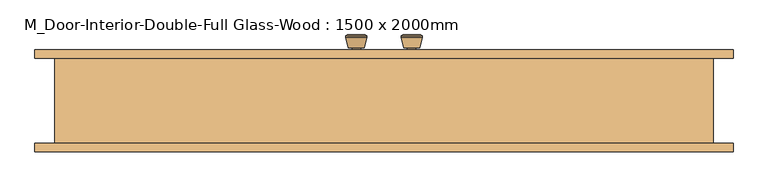
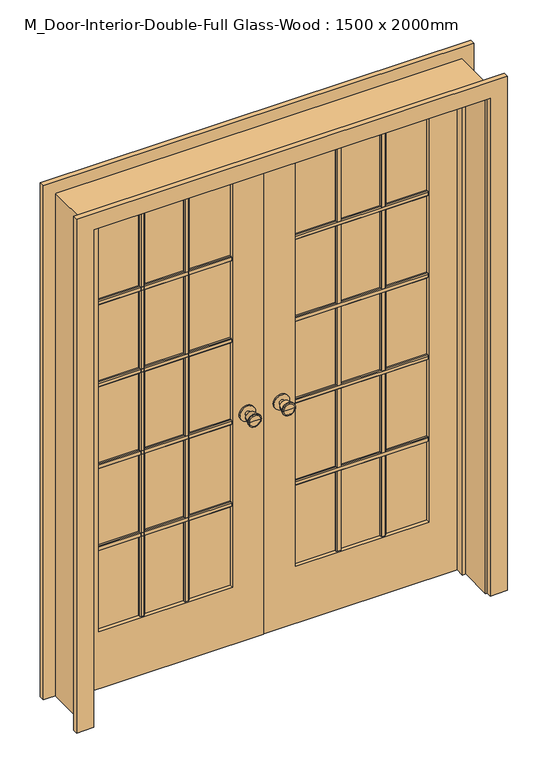
"""IFC4 building model written with IfcOpenShell, lengths in millimetres: door geometry, M_Door-Interior-Double-Full Glass-Wood : 1500 x 2000mm."""

import ifcopenshell
import ifcopenshell.guid

model = None  # the IFC model being written
_history = None  # IfcOwnerHistory: only IFC2X3 demands one
_inside = {}  # id of a spatial element -> (the spatial element, [elements in it])
_under = {}  # id of a project, library or spatial element -> (it, [spatial elements below it])
_declared = {}  # id of a project -> (the project, [libraries it declares])
_typed = {}  # id of a type object -> (the type object, [elements of that type])
_made_of = {}  # id of a material, layer set ... -> (it, [elements and type objects made of it])


def new_model(schema):
    """Start an empty IFC model of exactly this schema.

    Asked for "IFC4X3", IfcOpenShell would pick the latest addendum, in which some entities
    have other attributes; the version numbers below select the first issue.
    IFC2X3 requires an IfcOwnerHistory on every rooted entity: one is made here for all.
    """
    global model, _history
    if schema == "IFC4X3":
        model = ifcopenshell.file(schema_version=(4, 3, 0, 0))
    else:
        model = ifcopenshell.file(schema=schema)
    _inside.clear()
    _under.clear()
    _declared.clear()
    _typed.clear()
    _made_of.clear()
    _history = None
    if model.schema == "IFC2X3":
        org = make("IfcOrganization", Name="unknown")
        user = make(
            "IfcPersonAndOrganization",
            ThePerson=make("IfcPerson", FamilyName="unknown"),
            TheOrganization=org,
        )
        app = make(
            "IfcApplication",
            ApplicationDeveloper=org,
            Version="unknown",
            ApplicationFullName="unknown",
            ApplicationIdentifier="unknown",
        )
        _history = make(
            "IfcOwnerHistory",
            OwningUser=user,
            OwningApplication=app,
            ChangeAction="ADDED",
            CreationDate=0,
        )
    return model


def make(cls, **values):
    """One entity of the class cls with the attributes given. An attribute that is None is left unset."""
    return model.create_entity(
        cls, **{name: value for name, value in values.items() if value is not None}
    )


def rooted(cls, **values):
    """An entity with a GlobalId (a new one), such as an element, a storey or a relation."""
    return make(cls, GlobalId=ifcopenshell.guid.new(), OwnerHistory=_history, **values)


def si_unit(unit_type, name, prefix=None):
    """IfcSIUnit, for example si_unit("LENGTHUNIT", "METRE", prefix="MILLI")."""
    return make("IfcSIUnit", UnitType=unit_type, Prefix=prefix, Name=name)


def assignment(units):
    """IfcUnitAssignment: the units of a project."""
    return None if units is None else make("IfcUnitAssignment", Units=units)


def point(xyz):
    """IfcCartesianPoint."""
    return None if xyz is None else make("IfcCartesianPoint", Coordinates=xyz)


def direction(xyz):
    """IfcDirection."""
    return None if xyz is None else make("IfcDirection", DirectionRatios=xyz)


def frame(location, z_axis=None, x_axis=None):
    """IfcAxis2Placement3D, a coordinate frame: its origin and axes. An axis left out is left unset."""
    return make(
        "IfcAxis2Placement3D",
        Location=point(location),
        Axis=direction(z_axis),
        RefDirection=direction(x_axis),
    )


def frame_2d(location, x_axis=None):
    """IfcAxis2Placement2D, a coordinate frame in the plane: its origin and x axis."""
    return make(
        "IfcAxis2Placement2D", Location=point(location), RefDirection=direction(x_axis)
    )


def origin():
    """The frame at (0, 0, 0) with its axes left unset."""
    return frame((0.0, 0.0, 0.0))


def place(relative_to, where):
    """IfcLocalPlacement: puts the frame where relative to a parent placement (None: the world)."""
    return make(
        "IfcLocalPlacement", PlacementRelTo=relative_to, RelativePlacement=where
    )


def context(
    kind, dimensions, precision=None, world=None, true_north=None, identifier=None
):
    """IfcGeometricRepresentationContext, for example the 3D "Model" context."""
    return make(
        "IfcGeometricRepresentationContext",
        ContextIdentifier=identifier,
        ContextType=kind,
        CoordinateSpaceDimension=dimensions,
        Precision=precision,
        WorldCoordinateSystem=world,
        TrueNorth=true_north,
    )


def project(units=None, contexts=None):
    """IfcProject with its units and contexts."""
    return rooted(
        "IfcProject",
        Name="project",
        RepresentationContexts=contexts,
        UnitsInContext=assignment(units),
    )


def spatial(cls, under=None, at=None, **own):
    """A site, building, storey or space (cls), placed at a placement, below another one or the project."""
    s = rooted(cls, ObjectPlacement=at, **own)
    if under is not None:
        _under.setdefault(under.id(), (under, []))[1].append(s)
    return s


def polyline(points):
    """IfcPolyline through the points."""
    return make("IfcPolyline", Points=[point(p) for p in points])


def circle_curve(where, radius):
    """IfcCircle in the frame where."""
    return make("IfcCircle", Position=where, Radius=radius)


def trimmed(basis, trim1, trim2, sense, master):
    """IfcTrimmedCurve: the piece of a basis curve between two trims."""
    return make(
        "IfcTrimmedCurve",
        BasisCurve=basis,
        Trim1=trim1,
        Trim2=trim2,
        SenseAgreement=sense,
        MasterRepresentation=master,
    )


def segment(curve, same_sense, transition):
    """IfcCompositeCurveSegment."""
    return make(
        "IfcCompositeCurveSegment",
        Transition=transition,
        SameSense=same_sense,
        ParentCurve=curve,
    )


def composite_curve(segments, self_intersect=None):
    """IfcCompositeCurve: segments joined end to end."""
    return make("IfcCompositeCurve", Segments=segments, SelfIntersect=self_intersect)


def outline(outer, holes=None, kind="AREA"):
    """IfcArbitraryClosedProfileDef: a profile drawn as a closed curve; with holes, ...WithVoids."""
    if holes is None:
        return make("IfcArbitraryClosedProfileDef", ProfileType=kind, OuterCurve=outer)
    return make(
        "IfcArbitraryProfileDefWithVoids",
        ProfileType=kind,
        OuterCurve=outer,
        InnerCurves=holes,
    )


def extrude(swept, where, along, depth):
    """IfcExtrudedAreaSolid: the profile swept, set in the frame where, extruded along a direction by depth."""
    return make(
        "IfcExtrudedAreaSolid",
        SweptArea=swept,
        Position=where,
        ExtrudedDirection=direction(along),
        Depth=depth,
    )


def faces_of(points, faces, orient=None, outer=None):
    """IfcFace entities. A face is a list of loops; a loop is a list of indices into points, from 0.

    orient and outer hold one flag for each loop. By default every Orientation is true, the
    first loop of a face is its IfcFaceOuterBound and the others are IfcFaceBound.
    """
    made = []
    for i, loops in enumerate(faces):
        bounds = []
        for j, loop in enumerate(loops):
            is_outer = j == 0 if outer is None else outer[i][j]
            bounds.append(
                make(
                    "IfcFaceOuterBound" if is_outer else "IfcFaceBound",
                    Bound=make("IfcPolyLoop", Polygon=[points[k] for k in loop]),
                    Orientation=True if orient is None else orient[i][j],
                )
            )
        made.append(make("IfcFace", Bounds=bounds))
    return made


def faceted_brep(points, faces, orient=None, outer=None, voids=None):
    """IfcFacetedBrep: a solid bounded by flat faces; with voids (closed shells), ...WithVoids."""
    shared = [point(p) for p in points]
    hull = make("IfcClosedShell", CfsFaces=faces_of(shared, faces, orient, outer))
    if voids is None:
        return make("IfcFacetedBrep", Outer=hull)
    return make(
        "IfcFacetedBrepWithVoids",
        Outer=hull,
        Voids=[
            make(cls, CfsFaces=faces_of(shared, fs, o, b)) for cls, fs, o, b in voids
        ],
    )


def shape(context_of_items, identifier, shape_type, items):
    """IfcShapeRepresentation: the items that make up one representation, for example the "Body"."""
    return make(
        "IfcShapeRepresentation",
        ContextOfItems=context_of_items,
        RepresentationIdentifier=identifier,
        RepresentationType=shape_type,
        Items=items,
    )


def source(mapping_origin, context_of_items, identifier, shape_type, items):
    """IfcRepresentationMap: a shape defined once, which mapped items show again and again."""
    return make(
        "IfcRepresentationMap",
        MappingOrigin=mapping_origin,
        MappedRepresentation=shape(context_of_items, identifier, shape_type, items),
    )


def transform(
    local_origin,
    x_axis=None,
    y_axis=None,
    z_axis=None,
    scale=None,
    scale2=None,
    scale3=None,
    uniform=True,
):
    """IfcCartesianTransformationOperator3D, or its non-uniform kind. x_axis, y_axis, z_axis: its Axis1, 2, 3."""
    if uniform:
        return make(
            "IfcCartesianTransformationOperator3D",
            Axis1=direction(x_axis),
            Axis2=direction(y_axis),
            LocalOrigin=point(local_origin),
            Scale=scale,
            Axis3=direction(z_axis),
        )
    return make(
        "IfcCartesianTransformationOperator3DnonUniform",
        Axis1=direction(x_axis),
        Axis2=direction(y_axis),
        LocalOrigin=point(local_origin),
        Scale=scale,
        Axis3=direction(z_axis),
        Scale2=scale2,
        Scale3=scale3,
    )


def mapped(mapping_source, mapping_target):
    """IfcMappedItem: shows the shape of a source again, moved by a transform."""
    return make(
        "IfcMappedItem", MappingSource=mapping_source, MappingTarget=mapping_target
    )


def made_of(thing, what):
    """Note that an element or type object is made of a material, layer set ...; save() writes the relation."""
    if what is not None:
        _made_of.setdefault(what.id(), (what, []))[1].append(thing)
    return thing


def element(
    cls,
    number,
    at=None,
    inside=None,
    cuts=None,
    type_object=None,
    material=None,
    context=None,
    identifier="Body",
    shape_type=None,
    held_by="IfcProductDefinitionShape",
    body=None,
    shapes=None,
    **own,
):
    """One element of the class cls, such as IfcWall. Its Tag is "e" and its number.

    at: its placement. inside: the storey or other place that contains it. cuts: it is an
    opening in that element (IfcRelVoidsElement). A single representation is given by context,
    identifier, shape_type and body (its items); several are given by shapes. held_by: the class
    of the entity that holds the representations. save() writes the other relations.
    """
    e = rooted(cls, Tag="e%d" % number, ObjectPlacement=at, **own)
    if body is not None:
        shapes = [shape(context, identifier, shape_type, body)]
    if shapes is not None:
        e.Representation = make(held_by, Representations=shapes)
    if inside is not None:
        _inside.setdefault(inside.id(), (inside, []))[1].append(e)
    if cuts is not None:
        rooted(
            "IfcRelVoidsElement", RelatingBuildingElement=cuts, RelatedOpeningElement=e
        )
    if type_object is not None:
        _typed.setdefault(type_object.id(), (type_object, []))[1].append(e)
    return made_of(e, material)


def aggregate(whole, parts):
    """IfcRelAggregates: a whole, such as a stair, and the parts it consists of."""
    return rooted("IfcRelAggregates", RelatingObject=whole, RelatedObjects=parts)


def save(model, path):
    """Write the relations noted so far, then the file.

    IfcRelAggregates (storeys below a building ...), IfcRelContainedInSpatialStructure (elements
    in a storey), IfcRelDefinesByType, IfcRelAssociatesMaterial and IfcRelDeclares: one each for
    every whole, place, type object, material and project.
    """
    for whole, parts in _under.values():
        aggregate(whole, parts)
    for where, things in _inside.values():
        rooted(
            "IfcRelContainedInSpatialStructure",
            RelatedElements=things,
            RelatingStructure=where,
        )
    for kind, things in _typed.values():
        rooted("IfcRelDefinesByType", RelatedObjects=things, RelatingType=kind)
    for what, things in _made_of.values():
        rooted("IfcRelAssociatesMaterial", RelatedObjects=things, RelatingMaterial=what)
    for by, libraries in _declared.values():
        rooted("IfcRelDeclares", RelatingContext=by, RelatedDefinitions=libraries)
    model.write(path)


def plane_surface(at):
    """IfcPlane: the flat surface through the origin of the frame at, square to its z axis."""
    return make("IfcPlane", Position=at)


def cylinder_surface(at, radius):
    """IfcCylindricalSurface: all points at the distance radius from the z axis of the frame at."""
    return make("IfcCylindricalSurface", Position=at, Radius=radius)


def revolved_surface(curve, axis_point, axis_direction):
    """IfcSurfaceOfRevolution: the curve turned about the line through axis_point along axis_direction."""
    return make(
        "IfcSurfaceOfRevolution",
        SweptCurve=make("IfcArbitraryOpenProfileDef", ProfileType="CURVE", Curve=curve),
        AxisPosition=make("IfcAxis1Placement", Location=point(axis_point), Axis=direction(axis_direction)),
    )


def advanced_brep(points, edges, surfaces, faces):
    """IfcAdvancedBrep: a solid bounded by faces that lie on surfaces and meet in shared edges.

    An edge is (start, end): straight between two places in points (the first is 0);
    or (start, end, curve); or (start, end, curve, False) where it runs against its curve.
    A face is (place in surfaces, loops), or (place, loops, False) where it looks against
    its surface's normal. A loop lists edges by number (the first is 1), with a minus sign
    where the edge is run from its end to its start. The first loop is the outer one.
    """
    corners = [point(p) for p in points]
    vertices = [make("IfcVertexPoint", VertexGeometry=c) for c in corners]
    made = []
    for start, end, *more in edges:
        made.append(
            make(
                "IfcEdgeCurve",
                EdgeStart=vertices[start],
                EdgeEnd=vertices[end],
                EdgeGeometry=more[0] if more else make("IfcPolyline", Points=[corners[start], corners[end]]),
                SameSense=more[1] if len(more) > 1 else True,
            )
        )
    hull = []
    for where, loops, *sense in faces:
        bounds = []
        for j, loop in enumerate(loops):
            ring = [make("IfcOrientedEdge", EdgeElement=made[abs(k) - 1], Orientation=k > 0) for k in loop]
            bounds.append(
                make(
                    "IfcFaceOuterBound" if j == 0 else "IfcFaceBound",
                    Bound=make("IfcEdgeLoop", EdgeList=ring),
                    Orientation=True,
                )
            )
        hull.append(make("IfcAdvancedFace", Bounds=bounds, FaceSurface=surfaces[where], SameSense=sense[0] if sense else True))
    return make("IfcAdvancedBrep", Outer=make("IfcClosedShell", CfsFaces=hull))


def m_door_interior_double_full_glass_wood_1500_x_2000mm_af437330(model_context):
    return source(origin(), model_context, "Body", "SolidModel", [
        advanced_brep(
        [(-65.0, 102.825, 914.4), (-75.0, 102.825, 914.4), (-55.0, 102.825, 914.4), (-85.4758676, 151.825, 914.4), (-65.0, 151.825, 914.4), (-44.5241324, 151.825, 914.4), (-90.0, 149.9971319, 914.4), (-40.0, 149.9971319, 914.4), (-90.0, 146.5334537, 914.4), (-40.0, 146.5334537, 914.4), (-83.636236, 121.825, 914.4), (-46.363764, 121.825, 914.4), (-75.0, 121.825, 914.4), (-55.0, 121.825, 914.4)],
        [
            (0, 1),
            (1, 2, circle_curve(frame((-65.0, 102.825, 914.4), z_axis=(0.0, -1.0, 0.0), x_axis=(1.0, 0.0, 0.0)), 10.0)),
            (2, 0),
            (2, 1, circle_curve(frame((-65.0, 102.825, 914.4), z_axis=(0.0, -1.0, 0.0), x_axis=(1.0, 0.0, 0.0)), 10.0)),
            (3, 4),
            (4, 5),
            (5, 3, circle_curve(frame((-65.0, 151.825, 914.4), z_axis=(0.0, 1.0, 0.0), x_axis=(1.0, 0.0, 0.0)), 20.4758676)),
            (3, 5, circle_curve(frame((-65.0, 151.825, 914.4), z_axis=(0.0, 1.0, 0.0), x_axis=(1.0, 0.0, 0.0)), 20.4758676)),
            (6, 3),
            (5, 7),
            (7, 6, circle_curve(frame((-65.0, 149.9971319, 914.4), z_axis=(0.0, 1.0, 0.0), x_axis=(1.0, 0.0, 0.0)), 25.0)),
            (6, 7, circle_curve(frame((-65.0, 149.9971319, 914.4), z_axis=(0.0, 1.0, 0.0), x_axis=(1.0, 0.0, 0.0)), 25.0)),
            (8, 6),
            (7, 9),
            (9, 8, circle_curve(frame((-65.0, 146.5334537, 914.4), z_axis=(0.0, 1.0, 0.0), x_axis=(1.0, 0.0, 0.0)), 25.0)),
            (8, 9, circle_curve(frame((-65.0, 146.5334537, 914.4), z_axis=(0.0, 1.0, 0.0), x_axis=(1.0, 0.0, 0.0)), 25.0)),
            (10, 8),
            (9, 11),
            (11, 10, circle_curve(frame((-65.0, 121.825, 914.4), z_axis=(0.0, 1.0, 0.0), x_axis=(1.0, 0.0, 0.0)), 18.636236)),
            (10, 11, circle_curve(frame((-65.0, 121.825, 914.4), z_axis=(0.0, 1.0, 0.0), x_axis=(1.0, 0.0, 0.0)), 18.636236)),
            (12, 10),
            (11, 13),
            (13, 12, circle_curve(frame((-65.0, 121.825, 914.4), z_axis=(0.0, 1.0, 0.0), x_axis=(1.0, 0.0, 0.0)), 10.0)),
            (12, 13, circle_curve(frame((-65.0, 121.825, 914.4), z_axis=(0.0, 1.0, 0.0), x_axis=(1.0, 0.0, 0.0)), 10.0)),
            (1, 12),
            (13, 2),
        ],
        [
            plane_surface(frame((-65.0, 102.825, 914.4), z_axis=(0.0, -1.0, 0.0), x_axis=(1.0, 0.0, 0.0))),
            plane_surface(frame((-65.0, 151.825, 914.4), z_axis=(0.0, 1.0, 0.0), x_axis=(1.0, 0.0, 0.0))),
            revolved_surface(polyline([(-44.5241324, 151.825, 914.4), (-40.0, 149.9971319, 914.4)]), (-65.0, 102.825, 914.4), (0.0, -1.0, 0.0)),
            cylinder_surface(frame((-65.0, 102.825, 914.4), z_axis=(0.0, -1.0, 0.0), x_axis=(1.0, 0.0, 0.0)), 25.0),
            revolved_surface(polyline([(-40.0, 146.5334537, 914.4), (-46.363764, 121.825, 914.4)]), (-65.0, 102.825, 914.4), (0.0, -1.0, 0.0)),
            plane_surface(frame((-65.0, 121.825, 914.4), z_axis=(0.0, -1.0, 0.0), x_axis=(1.0, 0.0, 0.0))),
            cylinder_surface(frame((-65.0, 102.825, 914.4), z_axis=(0.0, -1.0, 0.0), x_axis=(1.0, 0.0, 0.0)), 10.0),
        ],
        [
            (0, [[1, 2, 3]]),
            (0, [[-3, 4, -1]]),
            (1, [[5, 6, 7]]),
            (1, [[-6, -5, 8]]),
            (2, [[9, -7, 10, 11]]),
            (2, [[-10, -8, -9, 12]]),
            (3, [[13, -11, 14, 15]]),
            (3, [[-14, -12, -13, 16]]),
            (4, [[17, -15, 18, 19]]),
            (4, [[-18, -16, -17, 20]]),
            (5, [[21, -19, 22, 23]]),
            (5, [[-22, -20, -21, 24]]),
            (6, [[25, -23, 26, -2]]),
            (6, [[-26, -24, -25, -4]]),
        ],
    ),
        extrude(outline(composite_curve([segment(trimmed(circle_curve(frame_2d((914.4, -65.0)), 30.0), [point((914.4, -35.0))], [point((914.4, -95.0))], False, "CARTESIAN"), True, "CONTINUOUS"), segment(trimmed(circle_curve(frame_2d((914.4, -65.0)), 30.0), [point((914.4, -95.0))], [point((914.4, -35.0))], False, "CARTESIAN"), True, "CONTINUOUS")], self_intersect=False)), frame((0.0, 96.825, 0.0), z_axis=(0.0, 1.0, 0.0), x_axis=(0.0, 0.0, 1.0)), (0.0, 0.0, 1.0), 6.0),
        advanced_brep(
        [(-65.0, 55.825, 914.4), (-55.0, 55.825, 914.4), (-75.0, 55.825, 914.4), (-85.4758676, 6.825, 914.4), (-44.5241324, 6.825, 914.4), (-65.0, 6.825, 914.4), (-90.0, 8.6528681, 914.4), (-40.0, 8.6528681, 914.4), (-90.0, 12.1165463, 914.4), (-40.0, 12.1165463, 914.4), (-83.636236, 36.825, 914.4), (-46.363764, 36.825, 914.4), (-75.0, 36.825, 914.4), (-55.0, 36.825, 914.4)],
        [
            (0, 1),
            (1, 2, circle_curve(frame((-65.0, 55.825, 914.4), z_axis=(0.0, 1.0, 0.0), x_axis=(1.0, 0.0, 0.0)), 10.0)),
            (2, 0),
            (2, 1, circle_curve(frame((-65.0, 55.825, 914.4), z_axis=(0.0, 1.0, 0.0), x_axis=(1.0, 0.0, 0.0)), 10.0)),
            (3, 4, circle_curve(frame((-65.0, 6.825, 914.4), z_axis=(0.0, -1.0, 0.0), x_axis=(1.0, 0.0, 0.0)), 20.4758676)),
            (4, 5),
            (5, 3),
            (4, 3, circle_curve(frame((-65.0, 6.825, 914.4), z_axis=(0.0, -1.0, 0.0), x_axis=(1.0, 0.0, 0.0)), 20.4758676)),
            (6, 7, circle_curve(frame((-65.0, 8.6528681, 914.4), z_axis=(0.0, -1.0, 0.0), x_axis=(1.0, 0.0, 0.0)), 25.0)),
            (7, 4),
            (3, 6),
            (7, 6, circle_curve(frame((-65.0, 8.6528681, 914.4), z_axis=(0.0, -1.0, 0.0), x_axis=(1.0, 0.0, 0.0)), 25.0)),
            (8, 9, circle_curve(frame((-65.0, 12.1165463, 914.4), z_axis=(0.0, -1.0, 0.0), x_axis=(1.0, 0.0, 0.0)), 25.0)),
            (9, 7),
            (6, 8),
            (9, 8, circle_curve(frame((-65.0, 12.1165463, 914.4), z_axis=(0.0, -1.0, 0.0), x_axis=(1.0, 0.0, 0.0)), 25.0)),
            (10, 11, circle_curve(frame((-65.0, 36.825, 914.4), z_axis=(0.0, -1.0, 0.0), x_axis=(1.0, 0.0, 0.0)), 18.636236)),
            (11, 9),
            (8, 10),
            (11, 10, circle_curve(frame((-65.0, 36.825, 914.4), z_axis=(0.0, -1.0, 0.0), x_axis=(1.0, 0.0, 0.0)), 18.636236)),
            (12, 13, circle_curve(frame((-65.0, 36.825, 914.4), z_axis=(0.0, -1.0, 0.0), x_axis=(1.0, 0.0, 0.0)), 10.0)),
            (13, 11),
            (10, 12),
            (13, 12, circle_curve(frame((-65.0, 36.825, 914.4), z_axis=(0.0, -1.0, 0.0), x_axis=(1.0, 0.0, 0.0)), 10.0)),
            (1, 13),
            (12, 2),
        ],
        [
            plane_surface(frame((-65.0, 55.825, 914.4), z_axis=(0.0, 1.0, 0.0), x_axis=(1.0, 0.0, 0.0))),
            plane_surface(frame((-65.0, 6.825, 914.4), z_axis=(0.0, -1.0, 0.0), x_axis=(1.0, 0.0, 0.0))),
            revolved_surface(polyline([(-44.5241324, 6.825, 914.4), (-40.0, 8.6528681, 914.4)]), (-65.0, 55.825, 914.4), (0.0, 1.0, 0.0)),
            cylinder_surface(frame((-65.0, 55.825, 914.4), z_axis=(0.0, 1.0, 0.0), x_axis=(1.0, 0.0, 0.0)), 25.0),
            revolved_surface(polyline([(-40.0, 12.1165463, 914.4), (-46.363764, 36.825, 914.4)]), (-65.0, 55.825, 914.4), (0.0, 1.0, 0.0)),
            plane_surface(frame((-65.0, 36.825, 914.4), z_axis=(0.0, 1.0, 0.0), x_axis=(1.0, 0.0, 0.0))),
            cylinder_surface(frame((-65.0, 55.825, 914.4), z_axis=(0.0, 1.0, 0.0), x_axis=(1.0, 0.0, 0.0)), 10.0),
        ],
        [
            (0, [[1, 2, 3]]),
            (0, [[-3, 4, -1]]),
            (1, [[5, 6, 7]]),
            (1, [[8, -7, -6]]),
            (2, [[9, 10, -5, 11]]),
            (2, [[12, -11, -8, -10]]),
            (3, [[13, 14, -9, 15]]),
            (3, [[16, -15, -12, -14]]),
            (4, [[17, 18, -13, 19]]),
            (4, [[20, -19, -16, -18]]),
            (5, [[21, 22, -17, 23]]),
            (5, [[24, -23, -20, -22]]),
            (6, [[-2, 25, -21, 26]]),
            (6, [[-4, -26, -24, -25]]),
        ],
    ),
        extrude(outline(composite_curve([segment(trimmed(circle_curve(frame_2d((914.4, -65.0)), 30.0), [point((914.4, -35.0))], [point((914.4, -95.0))], False, "CARTESIAN"), True, "CONTINUOUS"), segment(trimmed(circle_curve(frame_2d((914.4, -65.0)), 30.0), [point((914.4, -95.0))], [point((914.4, -35.0))], False, "CARTESIAN"), True, "CONTINUOUS")], self_intersect=False)), frame((0.0, 55.825, 0.0), z_axis=(0.0, 1.0, 0.0), x_axis=(0.0, 0.0, 1.0)), (0.0, 0.0, 1.0), 6.0),
        extrude(outline(polyline([(75.825, 1559.525), (75.825, 1540.475), (69.475, 1540.475), (66.3, 1543.65), (66.3, 1556.35), (69.475, 1559.525), (75.825, 1559.525)])), frame((120.0, 0.0, 0.0), z_axis=(1.0, 0.0, 0.0), x_axis=(0.0, 1.0, 0.0)), (0.0, 0.0, 1.0), 510.0),
        extrude(outline(polyline([(75.825, 1229.525), (75.825, 1210.475), (69.475, 1210.475), (66.3, 1213.65), (66.3, 1226.35), (69.475, 1229.525), (75.825, 1229.525)])), frame((120.0, 0.0, 0.0), z_axis=(1.0, 0.0, 0.0), x_axis=(0.0, 1.0, 0.0)), (0.0, 0.0, 1.0), 510.0),
        extrude(outline(polyline([(75.825, 899.525), (75.825, 880.475), (69.475, 880.475), (66.3, 883.65), (66.3, 896.35), (69.475, 899.525), (75.825, 899.525)])), frame((120.0, 0.0, 0.0), z_axis=(1.0, 0.0, 0.0), x_axis=(0.0, 1.0, 0.0)), (0.0, 0.0, 1.0), 510.0),
        extrude(outline(polyline([(75.825, 569.525), (75.825, 550.475), (69.475, 550.475), (66.3, 553.65), (66.3, 566.35), (69.475, 569.525), (75.825, 569.525)])), frame((120.0, 0.0, 0.0), z_axis=(1.0, 0.0, 0.0), x_axis=(0.0, 1.0, 0.0)), (0.0, 0.0, 1.0), 510.0),
        extrude(outline(polyline([(450.475, 75.825), (469.525, 75.825), (469.525, 69.475), (466.35, 66.3), (453.65, 66.3), (450.475, 69.475), (450.475, 75.825)])), frame((0.0, 0.0, 230.0), z_axis=(0.0, 0.0, 1.0), x_axis=(1.0, 0.0, 0.0)), (0.0, 0.0, 1.0), 1650.0),
        extrude(outline(polyline([(280.475, 75.825), (299.525, 75.825), (299.525, 69.475), (296.35, 66.3), (283.65, 66.3), (280.475, 69.475), (280.475, 75.825)])), frame((0.0, 0.0, 230.0), z_axis=(0.0, 0.0, 1.0), x_axis=(1.0, 0.0, 0.0)), (0.0, 0.0, 1.0), 1650.0),
        extrude(outline(polyline([(82.825, 1559.525), (89.175, 1559.525), (92.35, 1556.35), (92.35, 1543.65), (89.175, 1540.475), (82.825, 1540.475), (82.825, 1559.525)])), frame((-630.0, 0.0, 0.0), z_axis=(1.0, 0.0, 0.0), x_axis=(0.0, 1.0, 0.0)), (0.0, 0.0, 1.0), 510.0),
        extrude(outline(polyline([(82.825, 1229.525), (89.175, 1229.525), (92.35, 1226.35), (92.35, 1213.65), (89.175, 1210.475), (82.825, 1210.475), (82.825, 1229.525)])), frame((-630.0, 0.0, 0.0), z_axis=(1.0, 0.0, 0.0), x_axis=(0.0, 1.0, 0.0)), (0.0, 0.0, 1.0), 510.0),
        extrude(outline(polyline([(82.825, 899.525), (89.175, 899.525), (92.35, 896.35), (92.35, 883.65), (89.175, 880.475), (82.825, 880.475), (82.825, 899.525)])), frame((-630.0, 0.0, 0.0), z_axis=(1.0, 0.0, 0.0), x_axis=(0.0, 1.0, 0.0)), (0.0, 0.0, 1.0), 510.0),
        extrude(outline(polyline([(82.825, 569.525), (89.175, 569.525), (92.35, 566.35), (92.35, 553.65), (89.175, 550.475), (82.825, 550.475), (82.825, 569.525)])), frame((-630.0, 0.0, 0.0), z_axis=(1.0, 0.0, 0.0), x_axis=(0.0, 1.0, 0.0)), (0.0, 0.0, 1.0), 510.0),
        extrude(outline(polyline([(-299.525, 82.825), (-299.525, 89.175), (-296.35, 92.35), (-283.65, 92.35), (-280.475, 89.175), (-280.475, 82.825), (-299.525, 82.825)])), frame((0.0, 0.0, 230.0), z_axis=(0.0, 0.0, 1.0), x_axis=(1.0, 0.0, 0.0)), (0.0, 0.0, 1.0), 1650.0),
        extrude(outline(polyline([(-469.525, 82.825), (-469.525, 89.175), (-466.35, 92.35), (-453.65, 92.35), (-450.475, 89.175), (-450.475, 82.825), (-469.525, 82.825)])), frame((0.0, 0.0, 230.0), z_axis=(0.0, 0.0, 1.0), x_axis=(1.0, 0.0, 0.0)), (0.0, 0.0, 1.0), 1650.0),
        extrude(outline(polyline([(82.825, 1559.525), (89.175, 1559.525), (92.35, 1556.35), (92.35, 1543.65), (89.175, 1540.475), (82.825, 1540.475), (82.825, 1559.525)])), frame((120.0, 0.0, 0.0), z_axis=(1.0, 0.0, 0.0), x_axis=(0.0, 1.0, 0.0)), (0.0, 0.0, 1.0), 510.0),
        extrude(outline(polyline([(82.825, 1229.525), (89.175, 1229.525), (92.35, 1226.35), (92.35, 1213.65), (89.175, 1210.475), (82.825, 1210.475), (82.825, 1229.525)])), frame((120.0, 0.0, 0.0), z_axis=(1.0, 0.0, 0.0), x_axis=(0.0, 1.0, 0.0)), (0.0, 0.0, 1.0), 510.0),
        extrude(outline(polyline([(82.825, 899.525), (89.175, 899.525), (92.35, 896.35), (92.35, 883.65), (89.175, 880.475), (82.825, 880.475), (82.825, 899.525)])), frame((120.0, 0.0, 0.0), z_axis=(1.0, 0.0, 0.0), x_axis=(0.0, 1.0, 0.0)), (0.0, 0.0, 1.0), 510.0),
        extrude(outline(polyline([(82.825, 569.525), (89.175, 569.525), (92.35, 566.35), (92.35, 553.65), (89.175, 550.475), (82.825, 550.475), (82.825, 569.525)])), frame((120.0, 0.0, 0.0), z_axis=(1.0, 0.0, 0.0), x_axis=(0.0, 1.0, 0.0)), (0.0, 0.0, 1.0), 510.0),
        extrude(outline(polyline([(450.475, 82.825), (450.475, 89.175), (453.65, 92.35), (466.35, 92.35), (469.525, 89.175), (469.525, 82.825), (450.475, 82.825)])), frame((0.0, 0.0, 230.0), z_axis=(0.0, 0.0, 1.0), x_axis=(1.0, 0.0, 0.0)), (0.0, 0.0, 1.0), 1650.0),
        extrude(outline(polyline([(280.475, 82.825), (280.475, 89.175), (283.65, 92.35), (296.35, 92.35), (299.525, 89.175), (299.525, 82.825), (280.475, 82.825)])), frame((0.0, 0.0, 230.0), z_axis=(0.0, 0.0, 1.0), x_axis=(1.0, 0.0, 0.0)), (0.0, 0.0, 1.0), 1650.0),
        extrude(outline(polyline([(75.825, 1559.525), (75.825, 1540.475), (69.475, 1540.475), (66.3, 1543.65), (66.3, 1556.35), (69.475, 1559.525), (75.825, 1559.525)])), frame((-630.0, 0.0, 0.0), z_axis=(1.0, 0.0, 0.0), x_axis=(0.0, 1.0, 0.0)), (0.0, 0.0, 1.0), 510.0),
        extrude(outline(polyline([(75.825, 1229.525), (75.825, 1210.475), (69.475, 1210.475), (66.3, 1213.65), (66.3, 1226.35), (69.475, 1229.525), (75.825, 1229.525)])), frame((-630.0, 0.0, 0.0), z_axis=(1.0, 0.0, 0.0), x_axis=(0.0, 1.0, 0.0)), (0.0, 0.0, 1.0), 510.0),
        extrude(outline(polyline([(75.825, 899.525), (75.825, 880.475), (69.475, 880.475), (66.3, 883.65), (66.3, 896.35), (69.475, 899.525), (75.825, 899.525)])), frame((-630.0, 0.0, 0.0), z_axis=(1.0, 0.0, 0.0), x_axis=(0.0, 1.0, 0.0)), (0.0, 0.0, 1.0), 510.0),
        extrude(outline(polyline([(75.825, 569.525), (75.825, 550.475), (69.475, 550.475), (66.3, 553.65), (66.3, 566.35), (69.475, 569.525), (75.825, 569.525)])), frame((-630.0, 0.0, 0.0), z_axis=(1.0, 0.0, 0.0), x_axis=(0.0, 1.0, 0.0)), (0.0, 0.0, 1.0), 510.0),
        extrude(outline(polyline([(-299.525, 75.825), (-280.475, 75.825), (-280.475, 69.475), (-283.65, 66.3), (-296.35, 66.3), (-299.525, 69.475), (-299.525, 75.825)])), frame((0.0, 0.0, 230.0), z_axis=(0.0, 0.0, 1.0), x_axis=(1.0, 0.0, 0.0)), (0.0, 0.0, 1.0), 1650.0),
        extrude(outline(polyline([(-469.525, 75.825), (-450.475, 75.825), (-450.475, 69.475), (-453.65, 66.3), (-466.35, 66.3), (-469.525, 69.475), (-469.525, 75.825)])), frame((0.0, 0.0, 230.0), z_axis=(0.0, 0.0, 1.0), x_axis=(1.0, 0.0, 0.0)), (0.0, 0.0, 1.0), 1650.0),
        advanced_brep(
        [(65.0, 55.825, 914.4), (75.0, 55.825, 914.4), (55.0, 55.825, 914.4), (85.4758676, 6.825, 914.4), (65.0, 6.825, 914.4), (44.5241324, 6.825, 914.4), (90.0, 8.6528681, 914.4), (40.0, 8.6528681, 914.4), (90.0, 12.1165463, 914.4), (40.0, 12.1165463, 914.4), (83.636236, 36.825, 914.4), (46.363764, 36.825, 914.4), (75.0, 36.825, 914.4), (55.0, 36.825, 914.4)],
        [
            (0, 1),
            (1, 2, circle_curve(frame((65.0, 55.825, 914.4), z_axis=(0.0, 1.0, 0.0), x_axis=(-1.0, 0.0, 0.0)), 10.0)),
            (2, 0),
            (2, 1, circle_curve(frame((65.0, 55.825, 914.4), z_axis=(0.0, 1.0, 0.0), x_axis=(-1.0, 0.0, 0.0)), 10.0)),
            (3, 4),
            (4, 5),
            (5, 3, circle_curve(frame((65.0, 6.825, 914.4), z_axis=(0.0, -1.0, 0.0), x_axis=(-1.0, 0.0, 0.0)), 20.4758676)),
            (3, 5, circle_curve(frame((65.0, 6.825, 914.4), z_axis=(0.0, -1.0, 0.0), x_axis=(-1.0, 0.0, 0.0)), 20.4758676)),
            (6, 3),
            (5, 7),
            (7, 6, circle_curve(frame((65.0, 8.6528681, 914.4), z_axis=(0.0, -1.0, 0.0), x_axis=(-1.0, 0.0, 0.0)), 25.0)),
            (6, 7, circle_curve(frame((65.0, 8.6528681, 914.4), z_axis=(0.0, -1.0, 0.0), x_axis=(-1.0, 0.0, 0.0)), 25.0)),
            (8, 6),
            (7, 9),
            (9, 8, circle_curve(frame((65.0, 12.1165463, 914.4), z_axis=(0.0, -1.0, 0.0), x_axis=(-1.0, 0.0, 0.0)), 25.0)),
            (8, 9, circle_curve(frame((65.0, 12.1165463, 914.4), z_axis=(0.0, -1.0, 0.0), x_axis=(-1.0, 0.0, 0.0)), 25.0)),
            (10, 8),
            (9, 11),
            (11, 10, circle_curve(frame((65.0, 36.825, 914.4), z_axis=(0.0, -1.0, 0.0), x_axis=(-1.0, 0.0, 0.0)), 18.636236)),
            (10, 11, circle_curve(frame((65.0, 36.825, 914.4), z_axis=(0.0, -1.0, 0.0), x_axis=(-1.0, 0.0, 0.0)), 18.636236)),
            (12, 10),
            (11, 13),
            (13, 12, circle_curve(frame((65.0, 36.825, 914.4), z_axis=(0.0, -1.0, 0.0), x_axis=(-1.0, 0.0, 0.0)), 10.0)),
            (12, 13, circle_curve(frame((65.0, 36.825, 914.4), z_axis=(0.0, -1.0, 0.0), x_axis=(-1.0, 0.0, 0.0)), 10.0)),
            (1, 12),
            (13, 2),
        ],
        [
            plane_surface(frame((65.0, 55.825, 914.4), z_axis=(0.0, 1.0, 0.0), x_axis=(-1.0, 0.0, 0.0))),
            plane_surface(frame((65.0, 6.825, 914.4), z_axis=(0.0, -1.0, 0.0), x_axis=(-1.0, 0.0, 0.0))),
            revolved_surface(polyline([(44.5241324, 6.825, 914.4), (40.0, 8.6528681, 914.4)]), (65.0, 55.825, 914.4), (0.0, 1.0, 0.0)),
            cylinder_surface(frame((65.0, 55.825, 914.4), z_axis=(0.0, 1.0, 0.0), x_axis=(-1.0, 0.0, 0.0)), 25.0),
            revolved_surface(polyline([(40.0, 12.1165463, 914.4), (46.363764, 36.825, 914.4)]), (65.0, 55.825, 914.4), (0.0, 1.0, 0.0)),
            plane_surface(frame((65.0, 36.825, 914.4), z_axis=(0.0, 1.0, 0.0), x_axis=(-1.0, 0.0, 0.0))),
            cylinder_surface(frame((65.0, 55.825, 914.4), z_axis=(0.0, 1.0, 0.0), x_axis=(-1.0, 0.0, 0.0)), 10.0),
        ],
        [
            (0, [[1, 2, 3]]),
            (0, [[-3, 4, -1]]),
            (1, [[5, 6, 7]]),
            (1, [[-6, -5, 8]]),
            (2, [[9, -7, 10, 11]]),
            (2, [[-10, -8, -9, 12]]),
            (3, [[13, -11, 14, 15]]),
            (3, [[-14, -12, -13, 16]]),
            (4, [[17, -15, 18, 19]]),
            (4, [[-18, -16, -17, 20]]),
            (5, [[21, -19, 22, 23]]),
            (5, [[-22, -20, -21, 24]]),
            (6, [[25, -23, 26, -2]]),
            (6, [[-26, -24, -25, -4]]),
        ],
    ),
        extrude(outline(composite_curve([segment(trimmed(circle_curve(frame_2d((914.4, 65.0)), 30.0), [point((914.4, 35.0))], [point((914.4, 95.0))], False, "CARTESIAN"), True, "CONTINUOUS"), segment(trimmed(circle_curve(frame_2d((914.4, 65.0)), 30.0), [point((914.4, 95.0))], [point((914.4, 35.0))], False, "CARTESIAN"), True, "CONTINUOUS")], self_intersect=False)), frame((0.0, 55.825, 0.0), z_axis=(0.0, 1.0, 0.0), x_axis=(0.0, 0.0, 1.0)), (0.0, 0.0, 1.0), 6.0),
        advanced_brep(
        [(65.0, 102.825, 914.4), (55.0, 102.825, 914.4), (75.0, 102.825, 914.4), (85.4758676, 151.825, 914.4), (44.5241324, 151.825, 914.4), (65.0, 151.825, 914.4), (90.0, 149.9971319, 914.4), (40.0, 149.9971319, 914.4), (90.0, 146.5334537, 914.4), (40.0, 146.5334537, 914.4), (83.636236, 121.825, 914.4), (46.363764, 121.825, 914.4), (75.0, 121.825, 914.4), (55.0, 121.825, 914.4)],
        [
            (0, 1),
            (1, 2, circle_curve(frame((65.0, 102.825, 914.4), z_axis=(0.0, -1.0, 0.0), x_axis=(-1.0, 0.0, 0.0)), 10.0)),
            (2, 0),
            (2, 1, circle_curve(frame((65.0, 102.825, 914.4), z_axis=(0.0, -1.0, 0.0), x_axis=(-1.0, 0.0, 0.0)), 10.0)),
            (3, 4, circle_curve(frame((65.0, 151.825, 914.4), z_axis=(0.0, 1.0, 0.0), x_axis=(-1.0, 0.0, 0.0)), 20.4758676)),
            (4, 5),
            (5, 3),
            (4, 3, circle_curve(frame((65.0, 151.825, 914.4), z_axis=(0.0, 1.0, 0.0), x_axis=(-1.0, 0.0, 0.0)), 20.4758676)),
            (6, 7, circle_curve(frame((65.0, 149.9971319, 914.4), z_axis=(0.0, 1.0, 0.0), x_axis=(-1.0, 0.0, 0.0)), 25.0)),
            (7, 4),
            (3, 6),
            (7, 6, circle_curve(frame((65.0, 149.9971319, 914.4), z_axis=(0.0, 1.0, 0.0), x_axis=(-1.0, 0.0, 0.0)), 25.0)),
            (8, 9, circle_curve(frame((65.0, 146.5334537, 914.4), z_axis=(0.0, 1.0, 0.0), x_axis=(-1.0, 0.0, 0.0)), 25.0)),
            (9, 7),
            (6, 8),
            (9, 8, circle_curve(frame((65.0, 146.5334537, 914.4), z_axis=(0.0, 1.0, 0.0), x_axis=(-1.0, 0.0, 0.0)), 25.0)),
            (10, 11, circle_curve(frame((65.0, 121.825, 914.4), z_axis=(0.0, 1.0, 0.0), x_axis=(-1.0, 0.0, 0.0)), 18.636236)),
            (11, 9),
            (8, 10),
            (11, 10, circle_curve(frame((65.0, 121.825, 914.4), z_axis=(0.0, 1.0, 0.0), x_axis=(-1.0, 0.0, 0.0)), 18.636236)),
            (12, 13, circle_curve(frame((65.0, 121.825, 914.4), z_axis=(0.0, 1.0, 0.0), x_axis=(-1.0, 0.0, 0.0)), 10.0)),
            (13, 11),
            (10, 12),
            (13, 12, circle_curve(frame((65.0, 121.825, 914.4), z_axis=(0.0, 1.0, 0.0), x_axis=(-1.0, 0.0, 0.0)), 10.0)),
            (1, 13),
            (12, 2),
        ],
        [
            plane_surface(frame((65.0, 102.825, 914.4), z_axis=(0.0, -1.0, 0.0), x_axis=(-1.0, 0.0, 0.0))),
            plane_surface(frame((65.0, 151.825, 914.4), z_axis=(0.0, 1.0, 0.0), x_axis=(-1.0, 0.0, 0.0))),
            revolved_surface(polyline([(44.5241324, 151.825, 914.4), (40.0, 149.9971319, 914.4)]), (65.0, 102.825, 914.4), (0.0, -1.0, 0.0)),
            cylinder_surface(frame((65.0, 102.825, 914.4), z_axis=(0.0, -1.0, 0.0), x_axis=(-1.0, 0.0, 0.0)), 25.0),
            revolved_surface(polyline([(40.0, 146.5334537, 914.4), (46.363764, 121.825, 914.4)]), (65.0, 102.825, 914.4), (0.0, -1.0, 0.0)),
            plane_surface(frame((65.0, 121.825, 914.4), z_axis=(0.0, -1.0, 0.0), x_axis=(-1.0, 0.0, 0.0))),
            cylinder_surface(frame((65.0, 102.825, 914.4), z_axis=(0.0, -1.0, 0.0), x_axis=(-1.0, 0.0, 0.0)), 10.0),
        ],
        [
            (0, [[1, 2, 3]]),
            (0, [[-3, 4, -1]]),
            (1, [[5, 6, 7]]),
            (1, [[8, -7, -6]]),
            (2, [[9, 10, -5, 11]]),
            (2, [[12, -11, -8, -10]]),
            (3, [[13, 14, -9, 15]]),
            (3, [[16, -15, -12, -14]]),
            (4, [[17, 18, -13, 19]]),
            (4, [[20, -19, -16, -18]]),
            (5, [[21, 22, -17, 23]]),
            (5, [[24, -23, -20, -22]]),
            (6, [[-2, 25, -21, 26]]),
            (6, [[-4, -26, -24, -25]]),
        ],
    ),
        extrude(outline(composite_curve([segment(trimmed(circle_curve(frame_2d((914.4, 65.0)), 30.0), [point((914.4, 35.0))], [point((914.4, 95.0))], False, "CARTESIAN"), True, "CONTINUOUS"), segment(trimmed(circle_curve(frame_2d((914.4, 65.0)), 30.0), [point((914.4, 95.0))], [point((914.4, 35.0))], False, "CARTESIAN"), True, "CONTINUOUS")], self_intersect=False)), frame((0.0, 96.825, 0.0), z_axis=(0.0, 1.0, 0.0), x_axis=(0.0, 0.0, 1.0)), (0.0, 0.0, 1.0), 6.0),
        extrude(outline(polyline([(0.0, 756.35), (0.0, 821.35), (2071.35, 821.35), (2071.35, -821.35), (0.0, -821.35), (0.0, -756.35), (2006.35, -756.35), (2006.35, 756.35), (0.0, 756.35)])), frame((0.0, 96.825, 0.0), z_axis=(0.0, 1.0, 0.0), x_axis=(0.0, 0.0, 1.0)), (0.0, 0.0, 1.0), 20.0),
        extrude(outline(polyline([(0.0, 756.35), (0.0, 821.35), (2071.35, 821.35), (2071.35, -821.35), (0.0, -821.35), (0.0, -756.35), (2006.35, -756.35), (2006.35, 756.35), (0.0, 756.35)])), frame((0.0, -123.175, 0.0), z_axis=(0.0, 1.0, 0.0), x_axis=(0.0, 0.0, 1.0)), (0.0, 0.0, 1.0), 20.0),
        extrude(outline(polyline([(2000.0, -750.0), (0.0, -750.0), (0.0, -1.6019111), (2000.0, -1.6019111), (2000.0, -750.0)]), holes=[polyline([(230.0, -630.0), (1880.0, -630.0), (1880.0, -120.0), (230.0, -120.0), (230.0, -630.0)])]), frame((0.0, 61.825, 0.0), z_axis=(0.0, 1.0, 0.0), x_axis=(0.0, 0.0, 1.0)), (0.0, 0.0, 1.0), 35.0),
        extrude(outline(polyline([(0.0, 750.0), (2000.0, 750.0), (2000.0, 1.5875), (0.0, 1.5875), (0.0, 750.0)]), holes=[polyline([(1880.0, 120.0), (1880.0, 630.0), (230.0, 630.0), (230.0, 120.0), (1880.0, 120.0)])]), frame((0.0, 61.825, 0.0), z_axis=(0.0, 1.0, 0.0), x_axis=(0.0, 0.0, 1.0)), (0.0, 0.0, 1.0), 35.0),
        faceted_brep([(775.0, 96.825, 0.0), (775.0, -103.175, 0.0), (750.0, -103.175, 0.0), (750.0, 26.9, 0.0), (737.3, 26.9, 0.0), (737.3, 61.825, 0.0), (750.0, 61.825, 0.0), (750.0, 96.825, 0.0), (775.0, 96.825, 2025.0), (775.0, -103.175, 2025.0), (-775.0, -103.175, 2025.0), (-775.0, -103.175, 0.0), (-750.0, -103.175, 0.0), (-750.0, -103.175, 2000.0), (750.0, -103.175, 2000.0), (750.0, 26.9, 2000.0), (-750.0, 26.9, 2000.0), (-750.0, 26.9, 0.0), (-737.3, 26.9, 0.0), (-737.3, 26.9, 1987.3), (737.3, 26.9, 1987.3), (737.3, 61.825, 1987.3), (1.5875, 61.825, 1987.3), (-1.6019111, 61.825, 1987.3), (-737.3, 61.825, 1987.3), (-737.3, 61.825, 0.0), (-750.0, 61.825, 0.0), (-750.0, 61.825, 2000.0), (-1.6019111, 61.825, 2000.0), (1.5875, 61.825, 2000.0), (750.0, 61.825, 2000.0), (750.0, 96.825, 2000.0), (1.5875, 96.825, 2000.0), (-1.6019111, 96.825, 2000.0), (-750.0, 96.825, 2000.0), (-750.0, 96.825, 0.0), (-775.0, 96.825, 0.0), (-775.0, 96.825, 2025.0)], [[[0, 1, 2, 3, 4, 5, 6, 7]], [[1, 0, 8, 9]], [[2, 1, 9, 10, 11, 12, 13, 14]], [[3, 2, 14, 15]], [[4, 3, 15, 16, 17, 18, 19, 20]], [[5, 4, 20, 21]], [[6, 5, 21, 22, 23, 24, 25, 26, 27, 28, 29, 30]], [[7, 6, 30, 31]], [[0, 7, 31, 32, 33, 34, 35, 36, 37, 8]], [[9, 8, 37, 10]], [[14, 13, 16, 15]], [[20, 19, 24, 23, 22, 21]], [[31, 30, 29, 28, 27, 34, 33, 32]], [[12, 11, 36, 35, 26, 25, 18, 17]], [[11, 10, 37, 36]], [[13, 12, 17, 16]], [[19, 18, 25, 24]], [[27, 26, 35, 34]]]),
        extrude(outline(polyline([(630.0, 75.825), (120.0, 75.825), (120.0, 82.825), (630.0, 82.825), (630.0, 75.825)])), frame((0.0, 0.0, 230.0), z_axis=(0.0, 0.0, 1.0), x_axis=(1.0, 0.0, 0.0)), (0.0, 0.0, 1.0), 1650.0),
        extrude(outline(polyline([(-120.0, 75.825), (-630.0, 75.825), (-630.0, 82.825), (-120.0, 82.825), (-120.0, 75.825)])), frame((0.0, 0.0, 230.0), z_axis=(0.0, 0.0, 1.0), x_axis=(1.0, 0.0, 0.0)), (0.0, 0.0, 1.0), 1650.0),
    ])


if __name__ == "__main__":
    model = new_model("IFC4")
    model_context = context("Model", 3, world=origin())
    ifc_project = project(units=[si_unit("LENGTHUNIT", "METRE", prefix="MILLI")], contexts=[model_context])
    site = spatial("IfcSite", under=ifc_project)
    building = spatial("IfcBuilding", under=site)
    placement = place(None, origin())
    m_door_interior_double_full_glass_wood_1500_x_2000mm_shape = m_door_interior_double_full_glass_wood_1500_x_2000mm_af437330(model_context)
    element("IfcDoor", 1, ObjectType="M_Door-Interior-Double-Full Glass-Wood : 1500 x 2000mm", at=placement, inside=building, context=model_context, shape_type="MappedRepresentation", body=[
        mapped(m_door_interior_double_full_glass_wood_1500_x_2000mm_shape, transform((0.0, 0.0, 0.0), x_axis=(1.0, 0.0, 0.0), y_axis=(0.0, 1.0, 0.0), z_axis=(0.0, 0.0, 1.0))),
    ])
    save(model, "model.ifc")

# Revit data of these elements
# Project information
#   Organization Name = "// ORGANIZATION/NAME //"
#   Organization Description = "// ORGANIZATION/DESCRIPTION //"
#   Building Name = "// BUILDING/NAME //"
#   Author = "// AUTHOR //"
#   Project Issue Date = "// ISSUE DATE //"
#   Project Status = "// PROJECT/STATUS //"
#   Client Name = "// CLIENT/NAME //"
#   Project Address = "Enter address here"
#   Project Name = "// PROJECT/NAME //"
#   Project Number = "// PROJECT/NUMBER //"
# Type "M_Door-Interior-Double-Full Glass-Wood : 1500 x 2000mm"
#   Keynote = "Special wall: Keynote"
#   Model = "Special wall: Model"
#   Manufacturer = ""
#   URL = "Special wall: URL"
#   Type Mark = "41"
#   Assembly Code = "C1020300"
#   Analytic Construction = "French door, wood frame with single glass"
#   Top Rail = 120 mm
#   Thickness = 35 mm
#   Thermal Resistance (R) = 0.188367 (m²·K)/W
#   Swing Angle [instance default] = 90.00°
#   Stiles = 120 mm
#   Rough Width = 1550 mm
#   Rough Height = 2025 mm
#   Panel Width = 750 mm
#   Height = 2000 mm
#   Width = 1500 mm
#   Heat Transfer Coefficient (U) = 5.30918 W/(m²·K)
#   Bottom Rail = 230 mm
#   Show Grill [instance default] = yes
#   Trim Material = Cherry
#   Panel Material = Cherry
#   Frame Material = Cherry
#   Door Handle Material = Aluminum
#   Visual Light Transmittance = 0
#   Solar Heat Gain Coefficient = 0
#   Wall Closure = (empty or 0)
#   Function = (empty or 0)
# Element 1 (IfcDoor, "M_Door-Interior-Double-Full Glass-Wood : 1500 x 2000mm")
#   Materials on its faces: "Cherry", "Aluminum", "Glass"
# Materials
#   "Cherry": class "Wood", colour RGB 226 177 128, transparency 0, Description = "Prunus Serotina", Cost = 0
#   "Aluminum": class "Metal", colour RGB 247 247 247, transparency 0, Description = "Aluminum 6061", Cost = 0
#   "Glass": class "Glass", colour RGB 0 128 192, transparency 0.9, Description = "Soda Lime Glass", Cost = 0
